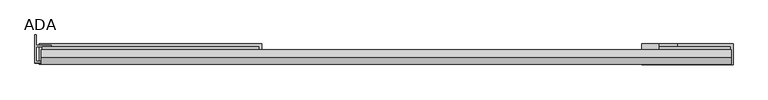
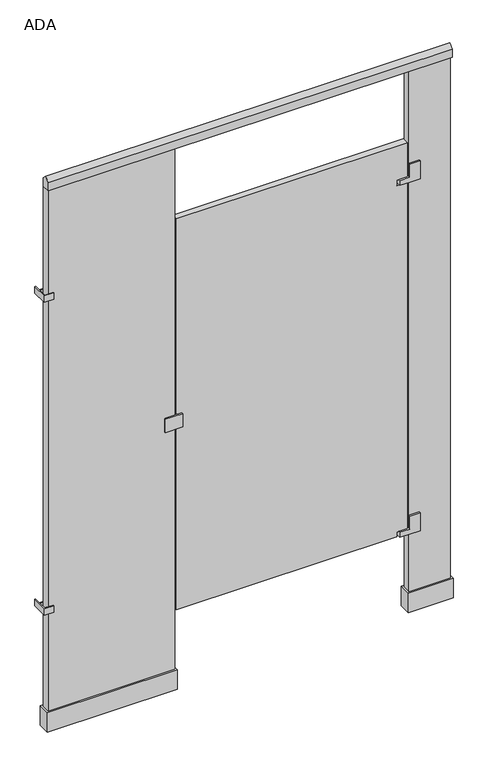
"""IFC4 building model written with IfcOpenShell, lengths in millimetres: proxy geometry, Toilet-Partition_Spec-Rite_Floor-Supported_Headrail : ADA."""

from ifc_helpers import new_model, si_unit, frame, origin, origin_with_axes, place, context, project, spatial, polyline, outline, extrude, source, transform, mapped, element, save


def ada_a7ce80af(model_context):
    return source(origin(), model_context, "Body", "SweptSolid", [
        extrude(outline(polyline([(-81.8439128, -2351.0927205), (-50.1871683, -2351.0927205), (-50.1871683, -2354.2677205), (-85.0189128, -2354.2677205), (-85.0189128, -2293.9427205), (-81.8886461, -2293.9427205), (-81.8886461, -2316.1677205), (-50.1871683, -2316.1677205), (-50.1871683, -2319.3427205), (-81.8439128, -2319.3427205), (-81.8439128, -2351.0927205)])), frame((0.0, 0.0, 1676.4), z_axis=(0.0, 0.0, 1.0), x_axis=(1.0, 0.0, 0.0)), (0.0, 0.0, 1.0), 25.4),
        extrude(outline(polyline([(-81.8439128, -2351.0927205), (-50.1871683, -2351.0927205), (-50.1871683, -2354.2677205), (-85.0189128, -2354.2677205), (-85.0189128, -2293.9427205), (-81.8886461, -2293.9427205), (-81.8886461, -2316.1677205), (-50.1871683, -2316.1677205), (-50.1871683, -2319.3427205), (-81.8439128, -2319.3427205), (-81.8439128, -2351.0927205)])), frame((0.0, 0.0, 457.2), z_axis=(0.0, 0.0, 1.0), x_axis=(1.0, 0.0, 0.0)), (0.0, 0.0, 1.0), 25.4),
        extrude(outline(polyline([(1413.5810872, -2351.0927205), (1261.1810872, -2351.0927205), (1261.1810872, -2319.3427205), (1413.5810872, -2319.3427205), (1413.5810872, -2351.0927205)])), origin_with_axes(), (0.0, 0.0, 1.0), 2133.6),
        extrude(outline(polyline([(397.5810872, -2351.0927205), (-69.1439128, -2351.0927205), (-69.1439128, -2319.3427205), (397.5810872, -2319.3427205), (397.5810872, -2351.0927205)])), origin_with_axes(), (0.0, 0.0, 1.0), 2133.6),
        extrude(outline(polyline([(359.4810872, -2357.4427205), (359.4810872, -2351.0927205), (422.9810872, -2351.0927205), (422.9810872, -2357.4427205), (359.4810872, -2357.4427205)])), frame((0.0, 0.0, 1015.4167184), z_axis=(0.0, 0.0, 1.0), x_axis=(1.0, 0.0, 0.0)), (0.0, 0.0, 1.0), 51.9665631),
        extrude(outline(polyline([(374.65, 1299.2810872), (374.65, 1261.1810872), (323.85, 1261.1810872), (323.85, 1223.0810872), (304.8, 1223.0810872), (304.8, 1299.2810872), (374.65, 1299.2810872)])), frame((0.0, -2357.4427205, 0.0), z_axis=(0.0, 1.0, 0.0), x_axis=(0.0, 0.0, 1.0)), (0.0, 0.0, 1.0), 44.4357849),
        extrude(outline(polyline([(1746.25, 1299.2810872), (1746.25, 1261.1810872), (1695.45, 1261.1810872), (1695.45, 1223.0810872), (1676.4, 1223.0810872), (1676.4, 1261.1810872), (1676.4, 1299.2810872), (1746.25, 1299.2810872)])), frame((0.0, -2357.4427205, 0.0), z_axis=(0.0, 1.0, 0.0), x_axis=(0.0, 0.0, 1.0)), (0.0, 0.0, 1.0), 44.4357849),
        extrude(outline(polyline([(304.8, 403.9310872), (304.8, 1216.7310872), (323.85, 1216.7310872), (323.85, 1254.8310872), (1674.426485, 1254.8310872), (1674.426485, 1216.7310872), (1695.45, 1216.7310872), (1695.45, 1254.8310872), (1828.8, 1254.8310872), (1828.8, 403.9310872), (304.8, 403.9310872)])), frame((0.0, -2351.0927205, 0.0), z_axis=(0.0, 1.0, 0.0), x_axis=(0.0, 0.0, 1.0)), (0.0, 0.0, 1.0), 25.4),
        extrude(outline(polyline([(-2357.4427205, 2139.95), (-2341.5677205, 2155.825), (-2325.6927205, 2139.95), (-2325.6927205, 2108.2), (-2357.4427205, 2108.2), (-2357.4427205, 2139.95)])), frame((-71.6931269, 0.0, 0.0), z_axis=(1.0, 0.0, 0.0), x_axis=(0.0, 1.0, 0.0)), (0.0, 0.0, 1.0), 1487.9739485),
        extrude(outline(polyline([(1254.8310872, -2357.6771735), (1254.8310872, -2313.0069356), (1419.9310872, -2313.0069356), (1419.9310872, -2357.6771735), (1254.8310872, -2357.6771735)])), origin_with_axes(), (0.0, 0.0, 1.0), 76.2),
        extrude(outline(polyline([(-75.4939128, -2357.317106), (-75.4939128, -2313.0516689), (403.9310872, -2313.0516689), (403.9310872, -2357.317106), (-75.4939128, -2357.317106)])), origin_with_axes(), (0.0, 0.0, 1.0), 76.2),
    ])


if __name__ == "__main__":
    model = new_model("IFC4")
    model_context = context("Model", 3, world=origin())
    ifc_project = project(units=[si_unit("LENGTHUNIT", "METRE", prefix="MILLI")], contexts=[model_context])
    site = spatial("IfcSite", under=ifc_project)
    building = spatial("IfcBuilding", under=site)
    placement = place(None, origin())
    ada_shape = ada_a7ce80af(model_context)
    element("IfcBuildingElementProxy", 1, Name="Toilet-Partition_Spec-Rite_Floor-Supported_Headrail : ADA", ObjectType="Toilet-Partition_Spec-Rite_Floor-Supported_Headrail : ADA", at=placement, inside=building, context=model_context, shape_type="MappedRepresentation", body=[
        mapped(ada_shape, transform((0.0, 0.0, 0.0), x_axis=(1.0, 0.0, 0.0), y_axis=(0.0, 1.0, 0.0), z_axis=(0.0, 0.0, 1.0))),
    ])
    save(model, "model.ifc")

# Revit data of these elements
# Type "Toilet-Partition_Spec-Rite_Floor-Supported_Headrail : ADA"
#   URL = "http://www.specritedesigns.com/"
#   UL Fire Rating [instance default] = ""
#   Manufacturer Phone - Toll Free = "877-249-6864"
#   Installation-Fabrication = "http://www.specritedesigns.com/partition_systems.aspx"
#   Green Building-LEED = "http://www.arcat.com/green/clients/leed_data_43944.html"
#   Specification = "http://www.arcat.com/sdspecs/htm/10150you.htm"
#   Send Message = "http://www.arcat.com/users.pl?action=UserEmail&company=Spec-Rite%20Designs%20LLC&coid=43944&rep=146&fax=314-771-4597&mf="
#   Sales Information = "http://www.specritedesigns.com/local_rep.aspx"
#   Revision = "R1_04/2010"
#   Product Properties = "http://www.arcat.com/bim/bim_info.pl?fn=Toilet-Partition_Spec-Rite_"
#   Product Data = "http://www.arcat.com/arcatcos/cos43/arc43944.html"
#   Model = "As Specified in 10 21 13"
#   Manufacturer's Notes = ""
#   Manufacturer Website = "http://www.specritedesigns.com/"
#   Manufacturer Phone = ""
#   Manufacturer Fax = "314-771-4597"
#   Manufacturer Address = "1054 Central Industrial Dr.; St. Louis; MO 63110"
#   Manufacturer = "Spec-Rite Designs LLC"
#   Keynote = "10 21 13"
#   Installation Phase = ""
#   Drawn By = "Robert S. Weygant, CSI, CDT, SCIP"
#   Core Material [instance default] = ""
#   Copyright = "2010, ARCAT, Inc."
#   Description = "As Specified in 10 21 13"
#   Construction Details = "http://www.specritedesigns.com/LinkClick.aspx?fileticket=c2fn%2bPpDPB4%3d&tabid=106"
#   Assembly Code = "C1010400"
#   topoffset = 0' - 0 1/4"
#   hngpnlconstrain [instance default] = 0' - 7 1/8"
#   hngpnl2 [instance default] = 0' - 1 1/8"
#   capoffset = 0' - 0 1/4"
#   Stile Thickness = 0' - 1 1/4"
#   Stall Width = 4' - 10"
#   Stall Depth = 5' - 0"
#   Pilaster Height = 7' - 0"
#   Panel Thickness = 0' - 1"
#   Panel Height = 5' - 0"
#   Front Panel Width_Strike Side = 1' - 6"
#   Reveal Clearance = 0' - 0 1/2"
#   Front Panel Width_Hinge Side = 0' - 6"
#   Door Width = 2' - 10"
#   Door Thickness = 0' - 1"
#   Distance from Floor to Panel = 1' - 0"
#   strkhdwr [instance default] = no
#   Warranty Duration (Years) = 0
#   Terminates at Wall_Strike Side [instance default] = no
#   Terminates at Wall_Hinge Side [instance default] = no
#   Return Rail - Strike Side [instance default] = yes
#   Return Rail - Hinge Side [instance default] = yes
#   Outswing [instance default] = no
#   Inswing [instance default] = yes
#   End Panel_Strike Side [instance default] = yes
#   Maintenance Schedule (Months) = 0
#   End Panel_Hinge Side [instance default] = yes
#   Expected Lifespan (Years) = 0
#   Brackets_Vertical = 2
#   Headrail Material = Aluminum - Extruded - Satin Anodized Finish
#   Hardware Type [instance default] = element 529356
#   Panel Material [instance default] = Phenolic Core - Color as Specified
#   Hardware Finish [instance default] = Stainless Steel - Type 304 #4 Brushed Finish
#   Type Comments = ""
# Element 1 (IfcBuildingElementProxy, "Toilet-Partition_Spec-Rite_Floor-Supported_Headrail : ADA")
#   hngpnlconstrain = 0' - 6"
#   hngpnl2 = 0' - 0 3/8"
#   Terminates at Wall_Strike Side = yes
#   Return Rail - Strike Side = no
#   Return Rail - Hinge Side = no
#   Outswing = yes
#   Inswing = no
#   End Panel_Strike Side = no
#   End Panel_Hinge Side = no
#   Materials on its faces: "Stainless Steel - Type 304 #4 Brushed Finish", "Phenolic Core - Color as Specified", "Aluminum - Extruded - Satin Anodized Finish"
# Materials
#   "Aluminum - Extruded - Satin Anodized Finish": class "Hardware Finishes", colour RGB 244 244 244, transparency 0, Model = "Aluminum - Extruded - Satin Anodized Finish", Description = "Aluminum - Extruded - Satin Anodized Finish", Cost = 0
#   "Phenolic Core - Color as Specified": class "Spec-Rite Partition Finishes", colour RGB 215 199 171, transparency 0, Keynote = "10 21 00", Model = "Phenolic Core - Color as Specified in 10 21 00", Manufacturer = "Spec-Rite Designs LLC", URL = "http://www.specritedesigns.com/", Description = "Phenolic Core - Color as Specified in 10 21 00", Cost = 0
#   "Stainless Steel - Type 304 #4 Brushed Finish": class "Hardware Finishes", colour RGB 189 187 185, transparency 0, Model = "Stainless Steel - Type 304 #4 Brushed Finish", Description = "Stainless Steel - Type 304 #4 Brushed Finish", Cost = 0
